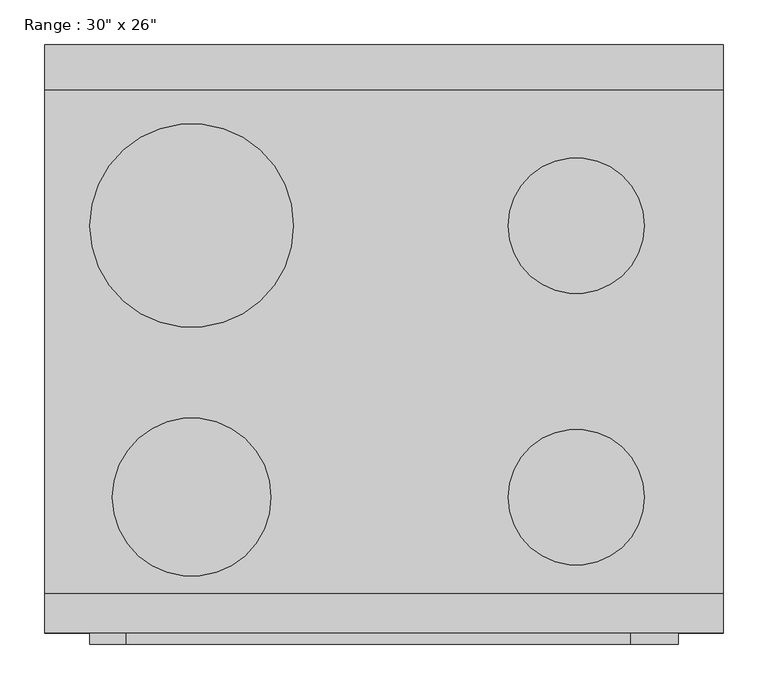
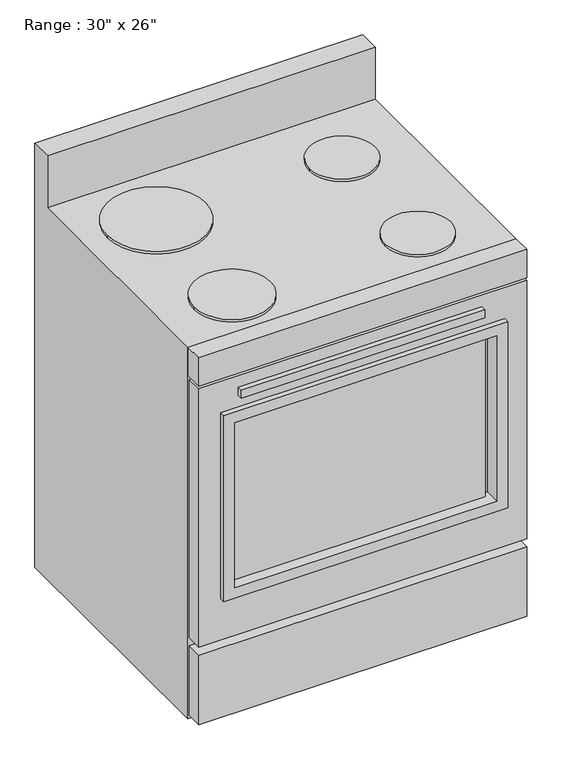
"""IFC4 building model written with IfcOpenShell, lengths in millimetres: proxy geometry."""

import ifcopenshell
import ifcopenshell.guid

model = None  # the IFC model being written
_history = None  # IfcOwnerHistory: only IFC2X3 demands one
_inside = {}  # id of a spatial element -> (the spatial element, [elements in it])
_under = {}  # id of a project, library or spatial element -> (it, [spatial elements below it])
_declared = {}  # id of a project -> (the project, [libraries it declares])
_typed = {}  # id of a type object -> (the type object, [elements of that type])
_made_of = {}  # id of a material, layer set ... -> (it, [elements and type objects made of it])


def new_model(schema):
    """Start an empty IFC model of exactly this schema.

    Asked for "IFC4X3", IfcOpenShell would pick the latest addendum, in which some entities
    have other attributes; the version numbers below select the first issue.
    IFC2X3 requires an IfcOwnerHistory on every rooted entity: one is made here for all.
    """
    global model, _history
    if schema == "IFC4X3":
        model = ifcopenshell.file(schema_version=(4, 3, 0, 0))
    else:
        model = ifcopenshell.file(schema=schema)
    _inside.clear()
    _under.clear()
    _declared.clear()
    _typed.clear()
    _made_of.clear()
    _history = None
    if model.schema == "IFC2X3":
        org = make("IfcOrganization", Name="unknown")
        user = make(
            "IfcPersonAndOrganization",
            ThePerson=make("IfcPerson", FamilyName="unknown"),
            TheOrganization=org,
        )
        app = make(
            "IfcApplication",
            ApplicationDeveloper=org,
            Version="unknown",
            ApplicationFullName="unknown",
            ApplicationIdentifier="unknown",
        )
        _history = make(
            "IfcOwnerHistory",
            OwningUser=user,
            OwningApplication=app,
            ChangeAction="ADDED",
            CreationDate=0,
        )
    return model


def make(cls, **values):
    """One entity of the class cls with the attributes given. An attribute that is None is left unset."""
    return model.create_entity(
        cls, **{name: value for name, value in values.items() if value is not None}
    )


def rooted(cls, **values):
    """An entity with a GlobalId (a new one), such as an element, a storey or a relation."""
    return make(cls, GlobalId=ifcopenshell.guid.new(), OwnerHistory=_history, **values)


def si_unit(unit_type, name, prefix=None):
    """IfcSIUnit, for example si_unit("LENGTHUNIT", "METRE", prefix="MILLI")."""
    return make("IfcSIUnit", UnitType=unit_type, Prefix=prefix, Name=name)


def assignment(units):
    """IfcUnitAssignment: the units of a project."""
    return None if units is None else make("IfcUnitAssignment", Units=units)


def point(xyz):
    """IfcCartesianPoint."""
    return None if xyz is None else make("IfcCartesianPoint", Coordinates=xyz)


def direction(xyz):
    """IfcDirection."""
    return None if xyz is None else make("IfcDirection", DirectionRatios=xyz)


def frame(location, z_axis=None, x_axis=None):
    """IfcAxis2Placement3D, a coordinate frame: its origin and axes. An axis left out is left unset."""
    return make(
        "IfcAxis2Placement3D",
        Location=point(location),
        Axis=direction(z_axis),
        RefDirection=direction(x_axis),
    )


def frame_2d(location, x_axis=None):
    """IfcAxis2Placement2D, a coordinate frame in the plane: its origin and x axis."""
    return make(
        "IfcAxis2Placement2D", Location=point(location), RefDirection=direction(x_axis)
    )


def origin():
    """The frame at (0, 0, 0) with its axes left unset."""
    return frame((0.0, 0.0, 0.0))


def place(relative_to, where):
    """IfcLocalPlacement: puts the frame where relative to a parent placement (None: the world)."""
    return make(
        "IfcLocalPlacement", PlacementRelTo=relative_to, RelativePlacement=where
    )


def context(
    kind, dimensions, precision=None, world=None, true_north=None, identifier=None
):
    """IfcGeometricRepresentationContext, for example the 3D "Model" context."""
    return make(
        "IfcGeometricRepresentationContext",
        ContextIdentifier=identifier,
        ContextType=kind,
        CoordinateSpaceDimension=dimensions,
        Precision=precision,
        WorldCoordinateSystem=world,
        TrueNorth=true_north,
    )


def project(units=None, contexts=None):
    """IfcProject with its units and contexts."""
    return rooted(
        "IfcProject",
        Name="project",
        RepresentationContexts=contexts,
        UnitsInContext=assignment(units),
    )


def spatial(cls, under=None, at=None, **own):
    """A site, building, storey or space (cls), placed at a placement, below another one or the project."""
    s = rooted(cls, ObjectPlacement=at, **own)
    if under is not None:
        _under.setdefault(under.id(), (under, []))[1].append(s)
    return s


def polyline(points):
    """IfcPolyline through the points."""
    return make("IfcPolyline", Points=[point(p) for p in points])


def circle_curve(where, radius):
    """IfcCircle in the frame where."""
    return make("IfcCircle", Position=where, Radius=radius)


def trimmed(basis, trim1, trim2, sense, master):
    """IfcTrimmedCurve: the piece of a basis curve between two trims."""
    return make(
        "IfcTrimmedCurve",
        BasisCurve=basis,
        Trim1=trim1,
        Trim2=trim2,
        SenseAgreement=sense,
        MasterRepresentation=master,
    )


def segment(curve, same_sense, transition):
    """IfcCompositeCurveSegment."""
    return make(
        "IfcCompositeCurveSegment",
        Transition=transition,
        SameSense=same_sense,
        ParentCurve=curve,
    )


def composite_curve(segments, self_intersect=None):
    """IfcCompositeCurve: segments joined end to end."""
    return make("IfcCompositeCurve", Segments=segments, SelfIntersect=self_intersect)


def outline(outer, holes=None, kind="AREA"):
    """IfcArbitraryClosedProfileDef: a profile drawn as a closed curve; with holes, ...WithVoids."""
    if holes is None:
        return make("IfcArbitraryClosedProfileDef", ProfileType=kind, OuterCurve=outer)
    return make(
        "IfcArbitraryProfileDefWithVoids",
        ProfileType=kind,
        OuterCurve=outer,
        InnerCurves=holes,
    )


def extrude(swept, where, along, depth):
    """IfcExtrudedAreaSolid: the profile swept, set in the frame where, extruded along a direction by depth."""
    return make(
        "IfcExtrudedAreaSolid",
        SweptArea=swept,
        Position=where,
        ExtrudedDirection=direction(along),
        Depth=depth,
    )


def faces_of(points, faces, orient=None, outer=None):
    """IfcFace entities. A face is a list of loops; a loop is a list of indices into points, from 0.

    orient and outer hold one flag for each loop. By default every Orientation is true, the
    first loop of a face is its IfcFaceOuterBound and the others are IfcFaceBound.
    """
    made = []
    for i, loops in enumerate(faces):
        bounds = []
        for j, loop in enumerate(loops):
            is_outer = j == 0 if outer is None else outer[i][j]
            bounds.append(
                make(
                    "IfcFaceOuterBound" if is_outer else "IfcFaceBound",
                    Bound=make("IfcPolyLoop", Polygon=[points[k] for k in loop]),
                    Orientation=True if orient is None else orient[i][j],
                )
            )
        made.append(make("IfcFace", Bounds=bounds))
    return made


def faceted_brep(points, faces, orient=None, outer=None, voids=None):
    """IfcFacetedBrep: a solid bounded by flat faces; with voids (closed shells), ...WithVoids."""
    shared = [point(p) for p in points]
    hull = make("IfcClosedShell", CfsFaces=faces_of(shared, faces, orient, outer))
    if voids is None:
        return make("IfcFacetedBrep", Outer=hull)
    return make(
        "IfcFacetedBrepWithVoids",
        Outer=hull,
        Voids=[
            make(cls, CfsFaces=faces_of(shared, fs, o, b)) for cls, fs, o, b in voids
        ],
    )


def shape(context_of_items, identifier, shape_type, items):
    """IfcShapeRepresentation: the items that make up one representation, for example the "Body"."""
    return make(
        "IfcShapeRepresentation",
        ContextOfItems=context_of_items,
        RepresentationIdentifier=identifier,
        RepresentationType=shape_type,
        Items=items,
    )


def source(mapping_origin, context_of_items, identifier, shape_type, items):
    """IfcRepresentationMap: a shape defined once, which mapped items show again and again."""
    return make(
        "IfcRepresentationMap",
        MappingOrigin=mapping_origin,
        MappedRepresentation=shape(context_of_items, identifier, shape_type, items),
    )


def transform(
    local_origin,
    x_axis=None,
    y_axis=None,
    z_axis=None,
    scale=None,
    scale2=None,
    scale3=None,
    uniform=True,
):
    """IfcCartesianTransformationOperator3D, or its non-uniform kind. x_axis, y_axis, z_axis: its Axis1, 2, 3."""
    if uniform:
        return make(
            "IfcCartesianTransformationOperator3D",
            Axis1=direction(x_axis),
            Axis2=direction(y_axis),
            LocalOrigin=point(local_origin),
            Scale=scale,
            Axis3=direction(z_axis),
        )
    return make(
        "IfcCartesianTransformationOperator3DnonUniform",
        Axis1=direction(x_axis),
        Axis2=direction(y_axis),
        LocalOrigin=point(local_origin),
        Scale=scale,
        Axis3=direction(z_axis),
        Scale2=scale2,
        Scale3=scale3,
    )


def mapped(mapping_source, mapping_target):
    """IfcMappedItem: shows the shape of a source again, moved by a transform."""
    return make(
        "IfcMappedItem", MappingSource=mapping_source, MappingTarget=mapping_target
    )


def made_of(thing, what):
    """Note that an element or type object is made of a material, layer set ...; save() writes the relation."""
    if what is not None:
        _made_of.setdefault(what.id(), (what, []))[1].append(thing)
    return thing


def element(
    cls,
    number,
    at=None,
    inside=None,
    cuts=None,
    type_object=None,
    material=None,
    context=None,
    identifier="Body",
    shape_type=None,
    held_by="IfcProductDefinitionShape",
    body=None,
    shapes=None,
    **own,
):
    """One element of the class cls, such as IfcWall. Its Tag is "e" and its number.

    at: its placement. inside: the storey or other place that contains it. cuts: it is an
    opening in that element (IfcRelVoidsElement). A single representation is given by context,
    identifier, shape_type and body (its items); several are given by shapes. held_by: the class
    of the entity that holds the representations. save() writes the other relations.
    """
    e = rooted(cls, Tag="e%d" % number, ObjectPlacement=at, **own)
    if body is not None:
        shapes = [shape(context, identifier, shape_type, body)]
    if shapes is not None:
        e.Representation = make(held_by, Representations=shapes)
    if inside is not None:
        _inside.setdefault(inside.id(), (inside, []))[1].append(e)
    if cuts is not None:
        rooted(
            "IfcRelVoidsElement", RelatingBuildingElement=cuts, RelatedOpeningElement=e
        )
    if type_object is not None:
        _typed.setdefault(type_object.id(), (type_object, []))[1].append(e)
    return made_of(e, material)


def aggregate(whole, parts):
    """IfcRelAggregates: a whole, such as a stair, and the parts it consists of."""
    return rooted("IfcRelAggregates", RelatingObject=whole, RelatedObjects=parts)


def save(model, path):
    """Write the relations noted so far, then the file.

    IfcRelAggregates (storeys below a building ...), IfcRelContainedInSpatialStructure (elements
    in a storey), IfcRelDefinesByType, IfcRelAssociatesMaterial and IfcRelDeclares: one each for
    every whole, place, type object, material and project.
    """
    for whole, parts in _under.values():
        aggregate(whole, parts)
    for where, things in _inside.values():
        rooted(
            "IfcRelContainedInSpatialStructure",
            RelatedElements=things,
            RelatingStructure=where,
        )
    for kind, things in _typed.values():
        rooted("IfcRelDefinesByType", RelatedObjects=things, RelatingType=kind)
    for what, things in _made_of.values():
        rooted("IfcRelAssociatesMaterial", RelatedObjects=things, RelatingMaterial=what)
    for by, libraries in _declared.values():
        rooted("IfcRelDeclares", RelatingContext=by, RelatedDefinitions=libraries)
    model.write(path)


def proxy_fbb4c072(model_context):
    return source(origin(), model_context, "Body", "SolidModel", [
        faceted_brep([(762.0, 660.4, 0.0), (0.0, 660.4, 0.0), (0.0, 660.4, 1041.4), (762.0, 660.4, 1041.4), (736.6, 660.4, 889.2220355), (25.4, 660.4, 889.2220355), (25.4, 660.4, 254.0), (736.6, 660.4, 254.0), (762.0, 44.45, 914.4), (0.0, 44.45, 914.4), (0.0, 44.45, 0.0), (762.0, 44.45, 0.0), (736.6, 44.45, 889.2220355), (736.6, 44.45, 254.0), (25.4, 44.45, 254.0), (25.4, 44.45, 889.2220355), (762.0, 609.6, 1041.4), (762.0, 609.6, 914.4), (0.0, 609.6, 914.4), (0.0, 609.6, 1041.4)], [[[0, 1, 2, 3], [4, 5, 6, 7]], [[8, 9, 10, 11], [12, 13, 14, 15]], [[0, 3, 16, 17, 8, 11]], [[1, 0, 11, 10]], [[2, 1, 10, 9, 18, 19]], [[9, 8, 17, 18]], [[5, 4, 12, 15]], [[6, 5, 15, 14]], [[7, 6, 14, 13]], [[4, 7, 13, 12]], [[16, 3, 2, 19]], [[17, 16, 19, 18]]]),
        extrude(outline(polyline([(657.225, -12.7), (91.687309, -12.7), (91.687309, 0.0), (657.225, 0.0), (657.225, -12.7)])), frame((0.0, 0.0, 791.2768639), z_axis=(0.0, 0.0, 1.0), x_axis=(1.0, 0.0, 0.0)), (0.0, 0.0, 1.0), 19.05),
        extrude(outline(polyline([(673.1, 12.7), (76.2, 12.7), (76.2, 19.05), (673.1, 19.05), (673.1, 12.7)])), frame((0.0, 0.0, 330.2), z_axis=(0.0, 0.0, 1.0), x_axis=(1.0, 0.0, 0.0)), (0.0, 0.0, 1.0), 406.4),
        extrude(outline(polyline([(762.0, 0.0), (0.0, 0.0), (0.0, 44.45), (762.0, 44.45), (762.0, 0.0)])), frame((0.0, 0.0, 844.7720355), z_axis=(0.0, 0.0, 1.0), x_axis=(1.0, 0.0, 0.0)), (0.0, 0.0, 1.0), 69.6279645),
        extrude(outline(polyline([(762.0, 711.2), (762.0, 50.8), (304.8, 50.8), (304.8, 711.2), (762.0, 711.2)]), holes=[polyline([(736.6, 685.8), (330.2, 685.8), (330.2, 76.2), (736.6, 76.2), (736.6, 685.8)])]), frame((0.0, -12.7, 0.0), z_axis=(0.0, 1.0, 0.0), x_axis=(0.0, 0.0, 1.0)), (0.0, 0.0, 1.0), 38.1),
        extrude(outline(composite_curve([segment(trimmed(circle_curve(frame_2d((165.1, 457.2)), 114.3), [point((50.8, 457.2))], [point((279.4, 457.2))], False, "CARTESIAN"), True, "CONTINUOUS"), segment(trimmed(circle_curve(frame_2d((165.1, 457.2)), 114.3), [point((279.4, 457.2))], [point((50.8, 457.2))], False, "CARTESIAN"), True, "CONTINUOUS")], self_intersect=False)), frame((0.0, 0.0, 914.4), z_axis=(0.0, 0.0, 1.0), x_axis=(1.0, 0.0, 0.0)), (0.0, 0.0, 1.0), 6.35),
        extrude(outline(composite_curve([segment(trimmed(circle_curve(frame_2d((596.9, 457.2)), 76.2), [point((520.7, 457.2))], [point((673.1, 457.2))], False, "CARTESIAN"), True, "CONTINUOUS"), segment(trimmed(circle_curve(frame_2d((596.9, 457.2)), 76.2), [point((673.1, 457.2))], [point((520.7, 457.2))], False, "CARTESIAN"), True, "CONTINUOUS")], self_intersect=False)), frame((0.0, 0.0, 914.4), z_axis=(0.0, 0.0, 1.0), x_axis=(1.0, 0.0, 0.0)), (0.0, 0.0, 1.0), 6.35),
        extrude(outline(composite_curve([segment(trimmed(circle_curve(frame_2d((596.9, 152.4)), 76.2), [point((520.7, 152.4))], [point((673.1, 152.4))], False, "CARTESIAN"), True, "CONTINUOUS"), segment(trimmed(circle_curve(frame_2d((596.9, 152.4)), 76.2), [point((673.1, 152.4))], [point((520.7, 152.4))], False, "CARTESIAN"), True, "CONTINUOUS")], self_intersect=False)), frame((0.0, 0.0, 914.4), z_axis=(0.0, 0.0, 1.0), x_axis=(1.0, 0.0, 0.0)), (0.0, 0.0, 1.0), 6.35),
        extrude(outline(composite_curve([segment(trimmed(circle_curve(frame_2d((165.1, 152.4)), 88.9), [point((76.2, 152.4))], [point((254.0, 152.4))], False, "CARTESIAN"), True, "CONTINUOUS"), segment(trimmed(circle_curve(frame_2d((165.1, 152.4)), 88.9), [point((254.0, 152.4))], [point((76.2, 152.4))], False, "CARTESIAN"), True, "CONTINUOUS")], self_intersect=False)), frame((0.0, 0.0, 914.4), z_axis=(0.0, 0.0, 1.0), x_axis=(1.0, 0.0, 0.0)), (0.0, 0.0, 1.0), 6.35),
        extrude(outline(polyline([(25.4, 660.4), (736.6, 660.4), (736.6, 635.0), (25.4, 635.0), (25.4, 660.4)])), frame((0.0, 0.0, 254.0), z_axis=(0.0, 0.0, 1.0), x_axis=(1.0, 0.0, 0.0)), (0.0, 0.0, 1.0), 635.2220355),
        extrude(outline(polyline([(838.4220355, 762.0), (838.4220355, 0.0), (203.2, 0.0), (203.2, 762.0), (838.4220355, 762.0)]), holes=[polyline([(762.0, 711.2), (304.8, 711.2), (304.8, 50.8), (762.0, 50.8), (762.0, 711.2)])]), frame((0.0, 0.0, 0.0), z_axis=(0.0, 1.0, 0.0), x_axis=(0.0, 0.0, 1.0)), (0.0, 0.0, 1.0), 38.1),
        extrude(outline(polyline([(762.0, 0.0), (0.0, 0.0), (0.0, 38.1), (762.0, 38.1), (762.0, 0.0)])), frame((0.0, 0.0, 12.7), z_axis=(0.0, 0.0, 1.0), x_axis=(1.0, 0.0, 0.0)), (0.0, 0.0, 1.0), 171.45),
    ])


if __name__ == "__main__":
    model = new_model("IFC4")
    model_context = context("Model", 3, world=origin())
    ifc_project = project(units=[si_unit("LENGTHUNIT", "METRE", prefix="MILLI")], contexts=[model_context])
    site = spatial("IfcSite", under=ifc_project)
    building = spatial("IfcBuilding", under=site)
    placement = place(None, origin())
    proxy_shape = proxy_fbb4c072(model_context)
    element("IfcBuildingElementProxy", 1, Name="Range : 30\" x 26\"", ObjectType="Range : 30\" x 26\"", at=placement, inside=building, context=model_context, shape_type="MappedRepresentation", body=[
        mapped(proxy_shape, transform((0.0, 0.0, 0.0), x_axis=(1.0, 0.0, 0.0), y_axis=(0.0, 1.0, 0.0), z_axis=(0.0, 0.0, 1.0))),
    ])
    save(model, "model.ifc")

# Revit data of these elements
# Type "Range : 30\" x 26\""
#   Assembly Code = "E1090400"
#   Depth = 2' - 2"
#   Width = 2' - 6"
#   Burner Material = Steel, Chrome Plated
#   Range Material = Steel, Paint Finish, Ivory, Matte
#   Default Elevation = 0
# Element 1 (IfcBuildingElementProxy, "Range : 30\" x 26\"")
#   Materials on its faces: "Steel, Paint Finish, Ivory, Matte", "Steel, Chrome Plated", "Glass"
# Materials
#   "Steel, Chrome Plated": class "Metal", colour RGB 244 244 244, transparency 0, Description = "Chromiuim plated steel", Cost = 0
#   "Steel, Paint Finish, Ivory, Matte": class "Metal", colour RGB 216 216 204, transparency 0, Description = "Steel, paint finish, ivory, matte", Cost = 0
#   "Glass": class "Glass", colour RGB 236 240 239, transparency 0.5, Description = "Soda Lime Glass", Cost = 0
